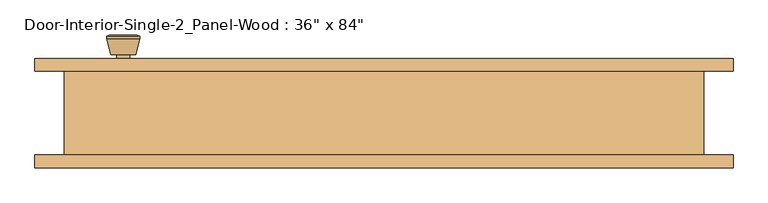
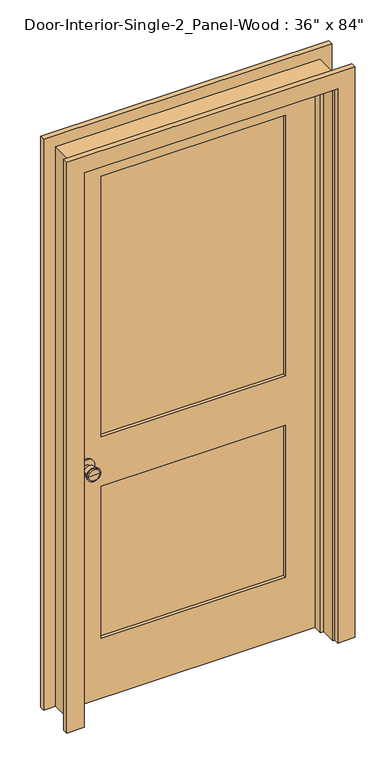
"""IFC4 building model written with IfcOpenShell, lengths in millimetres: door geometry."""

import ifcopenshell
import ifcopenshell.guid

model = None  # the IFC model being written
_history = None  # IfcOwnerHistory: only IFC2X3 demands one
_inside = {}  # id of a spatial element -> (the spatial element, [elements in it])
_under = {}  # id of a project, library or spatial element -> (it, [spatial elements below it])
_declared = {}  # id of a project -> (the project, [libraries it declares])
_typed = {}  # id of a type object -> (the type object, [elements of that type])
_made_of = {}  # id of a material, layer set ... -> (it, [elements and type objects made of it])


def new_model(schema):
    """Start an empty IFC model of exactly this schema.

    Asked for "IFC4X3", IfcOpenShell would pick the latest addendum, in which some entities
    have other attributes; the version numbers below select the first issue.
    IFC2X3 requires an IfcOwnerHistory on every rooted entity: one is made here for all.
    """
    global model, _history
    if schema == "IFC4X3":
        model = ifcopenshell.file(schema_version=(4, 3, 0, 0))
    else:
        model = ifcopenshell.file(schema=schema)
    _inside.clear()
    _under.clear()
    _declared.clear()
    _typed.clear()
    _made_of.clear()
    _history = None
    if model.schema == "IFC2X3":
        org = make("IfcOrganization", Name="unknown")
        user = make(
            "IfcPersonAndOrganization",
            ThePerson=make("IfcPerson", FamilyName="unknown"),
            TheOrganization=org,
        )
        app = make(
            "IfcApplication",
            ApplicationDeveloper=org,
            Version="unknown",
            ApplicationFullName="unknown",
            ApplicationIdentifier="unknown",
        )
        _history = make(
            "IfcOwnerHistory",
            OwningUser=user,
            OwningApplication=app,
            ChangeAction="ADDED",
            CreationDate=0,
        )
    return model


def make(cls, **values):
    """One entity of the class cls with the attributes given. An attribute that is None is left unset."""
    return model.create_entity(
        cls, **{name: value for name, value in values.items() if value is not None}
    )


def rooted(cls, **values):
    """An entity with a GlobalId (a new one), such as an element, a storey or a relation."""
    return make(cls, GlobalId=ifcopenshell.guid.new(), OwnerHistory=_history, **values)


def si_unit(unit_type, name, prefix=None):
    """IfcSIUnit, for example si_unit("LENGTHUNIT", "METRE", prefix="MILLI")."""
    return make("IfcSIUnit", UnitType=unit_type, Prefix=prefix, Name=name)


def assignment(units):
    """IfcUnitAssignment: the units of a project."""
    return None if units is None else make("IfcUnitAssignment", Units=units)


def point(xyz):
    """IfcCartesianPoint."""
    return None if xyz is None else make("IfcCartesianPoint", Coordinates=xyz)


def direction(xyz):
    """IfcDirection."""
    return None if xyz is None else make("IfcDirection", DirectionRatios=xyz)


def frame(location, z_axis=None, x_axis=None):
    """IfcAxis2Placement3D, a coordinate frame: its origin and axes. An axis left out is left unset."""
    return make(
        "IfcAxis2Placement3D",
        Location=point(location),
        Axis=direction(z_axis),
        RefDirection=direction(x_axis),
    )


def frame_2d(location, x_axis=None):
    """IfcAxis2Placement2D, a coordinate frame in the plane: its origin and x axis."""
    return make(
        "IfcAxis2Placement2D", Location=point(location), RefDirection=direction(x_axis)
    )


def origin():
    """The frame at (0, 0, 0) with its axes left unset."""
    return frame((0.0, 0.0, 0.0))


def place(relative_to, where):
    """IfcLocalPlacement: puts the frame where relative to a parent placement (None: the world)."""
    return make(
        "IfcLocalPlacement", PlacementRelTo=relative_to, RelativePlacement=where
    )


def context(
    kind, dimensions, precision=None, world=None, true_north=None, identifier=None
):
    """IfcGeometricRepresentationContext, for example the 3D "Model" context."""
    return make(
        "IfcGeometricRepresentationContext",
        ContextIdentifier=identifier,
        ContextType=kind,
        CoordinateSpaceDimension=dimensions,
        Precision=precision,
        WorldCoordinateSystem=world,
        TrueNorth=true_north,
    )


def project(units=None, contexts=None):
    """IfcProject with its units and contexts."""
    return rooted(
        "IfcProject",
        Name="project",
        RepresentationContexts=contexts,
        UnitsInContext=assignment(units),
    )


def spatial(cls, under=None, at=None, **own):
    """A site, building, storey or space (cls), placed at a placement, below another one or the project."""
    s = rooted(cls, ObjectPlacement=at, **own)
    if under is not None:
        _under.setdefault(under.id(), (under, []))[1].append(s)
    return s


def polyline(points):
    """IfcPolyline through the points."""
    return make("IfcPolyline", Points=[point(p) for p in points])


def circle_curve(where, radius):
    """IfcCircle in the frame where."""
    return make("IfcCircle", Position=where, Radius=radius)


def trimmed(basis, trim1, trim2, sense, master):
    """IfcTrimmedCurve: the piece of a basis curve between two trims."""
    return make(
        "IfcTrimmedCurve",
        BasisCurve=basis,
        Trim1=trim1,
        Trim2=trim2,
        SenseAgreement=sense,
        MasterRepresentation=master,
    )


def segment(curve, same_sense, transition):
    """IfcCompositeCurveSegment."""
    return make(
        "IfcCompositeCurveSegment",
        Transition=transition,
        SameSense=same_sense,
        ParentCurve=curve,
    )


def composite_curve(segments, self_intersect=None):
    """IfcCompositeCurve: segments joined end to end."""
    return make("IfcCompositeCurve", Segments=segments, SelfIntersect=self_intersect)


def outline(outer, holes=None, kind="AREA"):
    """IfcArbitraryClosedProfileDef: a profile drawn as a closed curve; with holes, ...WithVoids."""
    if holes is None:
        return make("IfcArbitraryClosedProfileDef", ProfileType=kind, OuterCurve=outer)
    return make(
        "IfcArbitraryProfileDefWithVoids",
        ProfileType=kind,
        OuterCurve=outer,
        InnerCurves=holes,
    )


def extrude(swept, where, along, depth):
    """IfcExtrudedAreaSolid: the profile swept, set in the frame where, extruded along a direction by depth."""
    return make(
        "IfcExtrudedAreaSolid",
        SweptArea=swept,
        Position=where,
        ExtrudedDirection=direction(along),
        Depth=depth,
    )


def faces_of(points, faces, orient=None, outer=None):
    """IfcFace entities. A face is a list of loops; a loop is a list of indices into points, from 0.

    orient and outer hold one flag for each loop. By default every Orientation is true, the
    first loop of a face is its IfcFaceOuterBound and the others are IfcFaceBound.
    """
    made = []
    for i, loops in enumerate(faces):
        bounds = []
        for j, loop in enumerate(loops):
            is_outer = j == 0 if outer is None else outer[i][j]
            bounds.append(
                make(
                    "IfcFaceOuterBound" if is_outer else "IfcFaceBound",
                    Bound=make("IfcPolyLoop", Polygon=[points[k] for k in loop]),
                    Orientation=True if orient is None else orient[i][j],
                )
            )
        made.append(make("IfcFace", Bounds=bounds))
    return made


def faceted_brep(points, faces, orient=None, outer=None, voids=None):
    """IfcFacetedBrep: a solid bounded by flat faces; with voids (closed shells), ...WithVoids."""
    shared = [point(p) for p in points]
    hull = make("IfcClosedShell", CfsFaces=faces_of(shared, faces, orient, outer))
    if voids is None:
        return make("IfcFacetedBrep", Outer=hull)
    return make(
        "IfcFacetedBrepWithVoids",
        Outer=hull,
        Voids=[
            make(cls, CfsFaces=faces_of(shared, fs, o, b)) for cls, fs, o, b in voids
        ],
    )


def shape(context_of_items, identifier, shape_type, items):
    """IfcShapeRepresentation: the items that make up one representation, for example the "Body"."""
    return make(
        "IfcShapeRepresentation",
        ContextOfItems=context_of_items,
        RepresentationIdentifier=identifier,
        RepresentationType=shape_type,
        Items=items,
    )


def source(mapping_origin, context_of_items, identifier, shape_type, items):
    """IfcRepresentationMap: a shape defined once, which mapped items show again and again."""
    return make(
        "IfcRepresentationMap",
        MappingOrigin=mapping_origin,
        MappedRepresentation=shape(context_of_items, identifier, shape_type, items),
    )


def transform(
    local_origin,
    x_axis=None,
    y_axis=None,
    z_axis=None,
    scale=None,
    scale2=None,
    scale3=None,
    uniform=True,
):
    """IfcCartesianTransformationOperator3D, or its non-uniform kind. x_axis, y_axis, z_axis: its Axis1, 2, 3."""
    if uniform:
        return make(
            "IfcCartesianTransformationOperator3D",
            Axis1=direction(x_axis),
            Axis2=direction(y_axis),
            LocalOrigin=point(local_origin),
            Scale=scale,
            Axis3=direction(z_axis),
        )
    return make(
        "IfcCartesianTransformationOperator3DnonUniform",
        Axis1=direction(x_axis),
        Axis2=direction(y_axis),
        LocalOrigin=point(local_origin),
        Scale=scale,
        Axis3=direction(z_axis),
        Scale2=scale2,
        Scale3=scale3,
    )


def mapped(mapping_source, mapping_target):
    """IfcMappedItem: shows the shape of a source again, moved by a transform."""
    return make(
        "IfcMappedItem", MappingSource=mapping_source, MappingTarget=mapping_target
    )


def made_of(thing, what):
    """Note that an element or type object is made of a material, layer set ...; save() writes the relation."""
    if what is not None:
        _made_of.setdefault(what.id(), (what, []))[1].append(thing)
    return thing


def element(
    cls,
    number,
    at=None,
    inside=None,
    cuts=None,
    type_object=None,
    material=None,
    context=None,
    identifier="Body",
    shape_type=None,
    held_by="IfcProductDefinitionShape",
    body=None,
    shapes=None,
    **own,
):
    """One element of the class cls, such as IfcWall. Its Tag is "e" and its number.

    at: its placement. inside: the storey or other place that contains it. cuts: it is an
    opening in that element (IfcRelVoidsElement). A single representation is given by context,
    identifier, shape_type and body (its items); several are given by shapes. held_by: the class
    of the entity that holds the representations. save() writes the other relations.
    """
    e = rooted(cls, Tag="e%d" % number, ObjectPlacement=at, **own)
    if body is not None:
        shapes = [shape(context, identifier, shape_type, body)]
    if shapes is not None:
        e.Representation = make(held_by, Representations=shapes)
    if inside is not None:
        _inside.setdefault(inside.id(), (inside, []))[1].append(e)
    if cuts is not None:
        rooted(
            "IfcRelVoidsElement", RelatingBuildingElement=cuts, RelatedOpeningElement=e
        )
    if type_object is not None:
        _typed.setdefault(type_object.id(), (type_object, []))[1].append(e)
    return made_of(e, material)


def aggregate(whole, parts):
    """IfcRelAggregates: a whole, such as a stair, and the parts it consists of."""
    return rooted("IfcRelAggregates", RelatingObject=whole, RelatedObjects=parts)


def save(model, path):
    """Write the relations noted so far, then the file.

    IfcRelAggregates (storeys below a building ...), IfcRelContainedInSpatialStructure (elements
    in a storey), IfcRelDefinesByType, IfcRelAssociatesMaterial and IfcRelDeclares: one each for
    every whole, place, type object, material and project.
    """
    for whole, parts in _under.values():
        aggregate(whole, parts)
    for where, things in _inside.values():
        rooted(
            "IfcRelContainedInSpatialStructure",
            RelatedElements=things,
            RelatingStructure=where,
        )
    for kind, things in _typed.values():
        rooted("IfcRelDefinesByType", RelatedObjects=things, RelatingType=kind)
    for what, things in _made_of.values():
        rooted("IfcRelAssociatesMaterial", RelatedObjects=things, RelatingMaterial=what)
    for by, libraries in _declared.values():
        rooted("IfcRelDeclares", RelatingContext=by, RelatedDefinitions=libraries)
    model.write(path)


def plane_surface(at):
    """IfcPlane: the flat surface through the origin of the frame at, square to its z axis."""
    return make("IfcPlane", Position=at)


def cylinder_surface(at, radius):
    """IfcCylindricalSurface: all points at the distance radius from the z axis of the frame at."""
    return make("IfcCylindricalSurface", Position=at, Radius=radius)


def revolved_surface(curve, axis_point, axis_direction):
    """IfcSurfaceOfRevolution: the curve turned about the line through axis_point along axis_direction."""
    return make(
        "IfcSurfaceOfRevolution",
        SweptCurve=make("IfcArbitraryOpenProfileDef", ProfileType="CURVE", Curve=curve),
        AxisPosition=make("IfcAxis1Placement", Location=point(axis_point), Axis=direction(axis_direction)),
    )


def advanced_brep(points, edges, surfaces, faces):
    """IfcAdvancedBrep: a solid bounded by faces that lie on surfaces and meet in shared edges.

    An edge is (start, end): straight between two places in points (the first is 0);
    or (start, end, curve); or (start, end, curve, False) where it runs against its curve.
    A face is (place in surfaces, loops), or (place, loops, False) where it looks against
    its surface's normal. A loop lists edges by number (the first is 1), with a minus sign
    where the edge is run from its end to its start. The first loop is the outer one.
    """
    corners = [point(p) for p in points]
    vertices = [make("IfcVertexPoint", VertexGeometry=c) for c in corners]
    made = []
    for start, end, *more in edges:
        made.append(
            make(
                "IfcEdgeCurve",
                EdgeStart=vertices[start],
                EdgeEnd=vertices[end],
                EdgeGeometry=more[0] if more else make("IfcPolyline", Points=[corners[start], corners[end]]),
                SameSense=more[1] if len(more) > 1 else True,
            )
        )
    hull = []
    for where, loops, *sense in faces:
        bounds = []
        for j, loop in enumerate(loops):
            ring = [make("IfcOrientedEdge", EdgeElement=made[abs(k) - 1], Orientation=k > 0) for k in loop]
            bounds.append(
                make(
                    "IfcFaceOuterBound" if j == 0 else "IfcFaceBound",
                    Bound=make("IfcEdgeLoop", EdgeList=ring),
                    Orientation=True,
                )
            )
        hull.append(make("IfcAdvancedFace", Bounds=bounds, FaceSurface=surfaces[where], SameSense=sense[0] if sense else True))
    return make("IfcAdvancedBrep", Outer=make("IfcClosedShell", CfsFaces=hull))


def door_9f0e9c7d(model_context):
    return source(origin(), model_context, "Body", "SolidModel", [
        advanced_brep(
        [(-393.7, 19.4, 914.4), (-383.7, 19.4, 914.4), (-403.7, 19.4, 914.4), (-373.2241324, -29.6, 914.4), (-393.7, -29.6, 914.4), (-414.1758676, -29.6, 914.4), (-368.7, -27.7721319, 914.4), (-418.7, -27.7721319, 914.4), (-368.7, -24.3084537, 914.4), (-418.7, -24.3084537, 914.4), (-375.063764, 0.4, 914.4), (-412.336236, 0.4, 914.4), (-383.7, 0.4, 914.4), (-403.7, 0.4, 914.4)],
        [
            (0, 1),
            (1, 2, circle_curve(frame((-393.7, 19.4, 914.4), z_axis=(0.0, 1.0, 0.0), x_axis=(-1.0, 0.0, 0.0)), 10.0)),
            (2, 0),
            (2, 1, circle_curve(frame((-393.7, 19.4, 914.4), z_axis=(0.0, 1.0, 0.0), x_axis=(-1.0, 0.0, 0.0)), 10.0)),
            (3, 4),
            (4, 5),
            (5, 3, circle_curve(frame((-393.7, -29.6, 914.4), z_axis=(0.0, -1.0, 0.0), x_axis=(-1.0, 0.0, 0.0)), 20.4758676)),
            (3, 5, circle_curve(frame((-393.7, -29.6, 914.4), z_axis=(0.0, -1.0, 0.0), x_axis=(-1.0, 0.0, 0.0)), 20.4758676)),
            (6, 3),
            (5, 7),
            (7, 6, circle_curve(frame((-393.7, -27.7721319, 914.4), z_axis=(0.0, -1.0, 0.0), x_axis=(-1.0, 0.0, 0.0)), 25.0)),
            (6, 7, circle_curve(frame((-393.7, -27.7721319, 914.4), z_axis=(0.0, -1.0, 0.0), x_axis=(-1.0, 0.0, 0.0)), 25.0)),
            (8, 6),
            (7, 9),
            (9, 8, circle_curve(frame((-393.7, -24.3084537, 914.4), z_axis=(0.0, -1.0, 0.0), x_axis=(-1.0, 0.0, 0.0)), 25.0)),
            (8, 9, circle_curve(frame((-393.7, -24.3084537, 914.4), z_axis=(0.0, -1.0, 0.0), x_axis=(-1.0, 0.0, 0.0)), 25.0)),
            (10, 8),
            (9, 11),
            (11, 10, circle_curve(frame((-393.7, 0.4, 914.4), z_axis=(0.0, -1.0, 0.0), x_axis=(-1.0, 0.0, 0.0)), 18.636236)),
            (10, 11, circle_curve(frame((-393.7, 0.4, 914.4), z_axis=(0.0, -1.0, 0.0), x_axis=(-1.0, 0.0, 0.0)), 18.636236)),
            (12, 10),
            (11, 13),
            (13, 12, circle_curve(frame((-393.7, 0.4, 914.4), z_axis=(0.0, -1.0, 0.0), x_axis=(-1.0, 0.0, 0.0)), 10.0)),
            (12, 13, circle_curve(frame((-393.7, 0.4, 914.4), z_axis=(0.0, -1.0, 0.0), x_axis=(-1.0, 0.0, 0.0)), 10.0)),
            (1, 12),
            (13, 2),
        ],
        [
            plane_surface(frame((-393.7, 19.4, 914.4), z_axis=(0.0, 1.0, 0.0), x_axis=(-1.0, 0.0, 0.0))),
            plane_surface(frame((-393.7, -29.6, 914.4), z_axis=(0.0, -1.0, 0.0), x_axis=(-1.0, 0.0, 0.0))),
            revolved_surface(polyline([(-414.1758676, -29.6, 914.4), (-418.7, -27.7721319, 914.4)]), (-393.7, 19.4, 914.4), (0.0, 1.0, 0.0)),
            cylinder_surface(frame((-393.7, 19.4, 914.4), z_axis=(0.0, 1.0, 0.0), x_axis=(-1.0, 0.0, 0.0)), 25.0),
            revolved_surface(polyline([(-418.7, -24.3084537, 914.4), (-412.336236, 0.4, 914.4)]), (-393.7, 19.4, 914.4), (0.0, 1.0, 0.0)),
            plane_surface(frame((-393.7, 0.4, 914.4), z_axis=(0.0, 1.0, 0.0), x_axis=(-1.0, 0.0, 0.0))),
            cylinder_surface(frame((-393.7, 19.4, 914.4), z_axis=(0.0, 1.0, 0.0), x_axis=(-1.0, 0.0, 0.0)), 10.0),
        ],
        [
            (0, [[1, 2, 3]]),
            (0, [[-3, 4, -1]]),
            (1, [[5, 6, 7]]),
            (1, [[-6, -5, 8]]),
            (2, [[9, -7, 10, 11]]),
            (2, [[-10, -8, -9, 12]]),
            (3, [[13, -11, 14, 15]]),
            (3, [[-14, -12, -13, 16]]),
            (4, [[17, -15, 18, 19]]),
            (4, [[-18, -16, -17, 20]]),
            (5, [[21, -19, 22, 23]]),
            (5, [[-22, -20, -21, 24]]),
            (6, [[25, -23, 26, -2]]),
            (6, [[-26, -24, -25, -4]]),
        ],
    ),
        extrude(outline(composite_curve([segment(trimmed(circle_curve(frame_2d((914.4, -393.7)), 30.0), [point((914.4, -423.7))], [point((914.4, -363.7))], False, "CARTESIAN"), True, "CONTINUOUS"), segment(trimmed(circle_curve(frame_2d((914.4, -393.7)), 30.0), [point((914.4, -363.7))], [point((914.4, -423.7))], False, "CARTESIAN"), True, "CONTINUOUS")], self_intersect=False)), frame((0.0, 19.4, 0.0), z_axis=(0.0, 1.0, 0.0), x_axis=(0.0, 0.0, 1.0)), (0.0, 0.0, 1.0), 6.0),
        advanced_brep(
        [(-393.7, 66.325, 914.4), (-403.7, 66.325, 914.4), (-383.7, 66.325, 914.4), (-373.2241324, 115.325, 914.4), (-414.1758676, 115.325, 914.4), (-393.7, 115.325, 914.4), (-368.7, 113.4971319, 914.4), (-418.7, 113.4971319, 914.4), (-368.7, 110.0334537, 914.4), (-418.7, 110.0334537, 914.4), (-375.063764, 85.325, 914.4), (-412.336236, 85.325, 914.4), (-383.7, 85.325, 914.4), (-403.7, 85.325, 914.4)],
        [
            (0, 1),
            (1, 2, circle_curve(frame((-393.7, 66.325, 914.4), z_axis=(0.0, -1.0, 0.0), x_axis=(-1.0, 0.0, 0.0)), 10.0)),
            (2, 0),
            (2, 1, circle_curve(frame((-393.7, 66.325, 914.4), z_axis=(0.0, -1.0, 0.0), x_axis=(-1.0, 0.0, 0.0)), 10.0)),
            (3, 4, circle_curve(frame((-393.7, 115.325, 914.4), z_axis=(0.0, 1.0, 0.0), x_axis=(-1.0, 0.0, 0.0)), 20.4758676)),
            (4, 5),
            (5, 3),
            (4, 3, circle_curve(frame((-393.7, 115.325, 914.4), z_axis=(0.0, 1.0, 0.0), x_axis=(-1.0, 0.0, 0.0)), 20.4758676)),
            (6, 7, circle_curve(frame((-393.7, 113.4971319, 914.4), z_axis=(0.0, 1.0, 0.0), x_axis=(-1.0, 0.0, 0.0)), 25.0)),
            (7, 4),
            (3, 6),
            (7, 6, circle_curve(frame((-393.7, 113.4971319, 914.4), z_axis=(0.0, 1.0, 0.0), x_axis=(-1.0, 0.0, 0.0)), 25.0)),
            (8, 9, circle_curve(frame((-393.7, 110.0334537, 914.4), z_axis=(0.0, 1.0, 0.0), x_axis=(-1.0, 0.0, 0.0)), 25.0)),
            (9, 7),
            (6, 8),
            (9, 8, circle_curve(frame((-393.7, 110.0334537, 914.4), z_axis=(0.0, 1.0, 0.0), x_axis=(-1.0, 0.0, 0.0)), 25.0)),
            (10, 11, circle_curve(frame((-393.7, 85.325, 914.4), z_axis=(0.0, 1.0, 0.0), x_axis=(-1.0, 0.0, 0.0)), 18.636236)),
            (11, 9),
            (8, 10),
            (11, 10, circle_curve(frame((-393.7, 85.325, 914.4), z_axis=(0.0, 1.0, 0.0), x_axis=(-1.0, 0.0, 0.0)), 18.636236)),
            (12, 13, circle_curve(frame((-393.7, 85.325, 914.4), z_axis=(0.0, 1.0, 0.0), x_axis=(-1.0, 0.0, 0.0)), 10.0)),
            (13, 11),
            (10, 12),
            (13, 12, circle_curve(frame((-393.7, 85.325, 914.4), z_axis=(0.0, 1.0, 0.0), x_axis=(-1.0, 0.0, 0.0)), 10.0)),
            (1, 13),
            (12, 2),
        ],
        [
            plane_surface(frame((-393.7, 66.325, 914.4), z_axis=(0.0, -1.0, 0.0), x_axis=(-1.0, 0.0, 0.0))),
            plane_surface(frame((-393.7, 115.325, 914.4), z_axis=(0.0, 1.0, 0.0), x_axis=(-1.0, 0.0, 0.0))),
            revolved_surface(polyline([(-414.1758676, 115.325, 914.4), (-418.7, 113.4971319, 914.4)]), (-393.7, 66.325, 914.4), (0.0, -1.0, 0.0)),
            cylinder_surface(frame((-393.7, 66.325, 914.4), z_axis=(0.0, -1.0, 0.0), x_axis=(-1.0, 0.0, 0.0)), 25.0),
            revolved_surface(polyline([(-418.7, 110.0334537, 914.4), (-412.336236, 85.325, 914.4)]), (-393.7, 66.325, 914.4), (0.0, -1.0, 0.0)),
            plane_surface(frame((-393.7, 85.325, 914.4), z_axis=(0.0, -1.0, 0.0), x_axis=(-1.0, 0.0, 0.0))),
            cylinder_surface(frame((-393.7, 66.325, 914.4), z_axis=(0.0, -1.0, 0.0), x_axis=(-1.0, 0.0, 0.0)), 10.0),
        ],
        [
            (0, [[1, 2, 3]]),
            (0, [[-3, 4, -1]]),
            (1, [[5, 6, 7]]),
            (1, [[8, -7, -6]]),
            (2, [[9, 10, -5, 11]]),
            (2, [[12, -11, -8, -10]]),
            (3, [[13, 14, -9, 15]]),
            (3, [[16, -15, -12, -14]]),
            (4, [[17, 18, -13, 19]]),
            (4, [[20, -19, -16, -18]]),
            (5, [[21, 22, -17, 23]]),
            (5, [[24, -23, -20, -22]]),
            (6, [[-2, 25, -21, 26]]),
            (6, [[-4, -26, -24, -25]]),
        ],
    ),
        extrude(outline(composite_curve([segment(trimmed(circle_curve(frame_2d((914.4, -393.7)), 30.0), [point((914.4, -423.7))], [point((914.4, -363.7))], False, "CARTESIAN"), True, "CONTINUOUS"), segment(trimmed(circle_curve(frame_2d((914.4, -393.7)), 30.0), [point((914.4, -363.7))], [point((914.4, -423.7))], False, "CARTESIAN"), True, "CONTINUOUS")], self_intersect=False)), frame((0.0, 60.325, 0.0), z_axis=(0.0, 1.0, 0.0), x_axis=(0.0, 0.0, 1.0)), (0.0, 0.0, 1.0), 6.0),
        extrude(outline(polyline([(336.55, 37.0416667), (-336.55, 37.0416667), (-336.55, 48.6833333), (336.55, 48.6833333), (336.55, 37.0416667)])), frame((0.0, 0.0, 1009.65), z_axis=(0.0, 0.0, 1.0), x_axis=(1.0, 0.0, 0.0)), (0.0, 0.0, 1.0), 1004.8875),
        extrude(outline(polyline([(336.55, 37.0416667), (-336.55, 37.0416667), (-336.55, 48.6833333), (336.55, 48.6833333), (336.55, 37.0416667)])), frame((0.0, 0.0, 231.775), z_axis=(0.0, 0.0, 1.0), x_axis=(1.0, 0.0, 0.0)), (0.0, 0.0, 1.0), 587.375),
        extrude(outline(polyline([(2133.6, -457.2), (0.0, -457.2), (0.0, 457.2), (2133.6, 457.2), (2133.6, -457.2)]), holes=[polyline([(2014.5375, -336.55), (2014.5375, 336.55), (1009.65, 336.55), (1009.65, -336.55), (2014.5375, -336.55)]), polyline([(819.15, -336.55), (819.15, 336.55), (231.775, 336.55), (231.775, -336.55), (819.15, -336.55)])]), frame((0.0, 25.4, 0.0), z_axis=(0.0, 1.0, 0.0), x_axis=(0.0, 0.0, 1.0)), (0.0, 0.0, 1.0), 34.925),
        faceted_brep([(482.6, 60.325, 0.0), (482.6, -66.675, 0.0), (457.2, -66.675, 0.0), (457.2, -9.525, 0.0), (444.5, -9.525, 0.0), (444.5, 25.4, 0.0), (457.2, 25.4, 0.0), (457.2, 60.325, 0.0), (482.6, 60.325, 2159.0), (482.6, -66.675, 2159.0), (-482.6, -66.675, 2159.0), (-482.6, -66.675, 0.0), (-457.2, -66.675, 0.0), (-457.2, -66.675, 2133.6), (457.2, -66.675, 2133.6), (457.2, -9.525, 2133.6), (-457.2, -9.525, 2133.6), (-457.2, -9.525, 0.0), (-444.5, -9.525, 0.0), (-444.5, -9.525, 2120.9), (444.5, -9.525, 2120.9), (444.5, 25.4, 2120.9), (-444.5, 25.4, 2120.9), (-444.5, 25.4, 0.0), (-457.2, 25.4, 0.0), (-457.2, 25.4, 2133.6), (457.2, 25.4, 2133.6), (457.2, 60.325, 2133.6), (-457.2, 60.325, 2133.6), (-457.2, 60.325, 0.0), (-482.6, 60.325, 0.0), (-482.6, 60.325, 2159.0)], [[[0, 1, 2, 3, 4, 5, 6, 7]], [[1, 0, 8, 9]], [[2, 1, 9, 10, 11, 12, 13, 14]], [[3, 2, 14, 15]], [[4, 3, 15, 16, 17, 18, 19, 20]], [[5, 4, 20, 21]], [[6, 5, 21, 22, 23, 24, 25, 26]], [[7, 6, 26, 27]], [[0, 7, 27, 28, 29, 30, 31, 8]], [[9, 8, 31, 10]], [[15, 14, 13, 16]], [[21, 20, 19, 22]], [[27, 26, 25, 28]], [[30, 29, 24, 23, 18, 17, 12, 11]], [[10, 31, 30, 11]], [[16, 13, 12, 17]], [[22, 19, 18, 23]], [[28, 25, 24, 29]]]),
        extrude(outline(polyline([(0.0, 463.55), (0.0, 527.05), (2203.45, 527.05), (2203.45, -527.05), (0.0, -527.05), (0.0, -463.55), (2139.95, -463.55), (2139.95, 463.55), (0.0, 463.55)])), frame((0.0, -85.725, 0.0), z_axis=(0.0, 1.0, 0.0), x_axis=(0.0, 0.0, 1.0)), (0.0, 0.0, 1.0), 19.05),
        extrude(outline(polyline([(0.0, 463.55), (0.0, 527.05), (2203.45, 527.05), (2203.45, -527.05), (0.0, -527.05), (0.0, -463.55), (2139.95, -463.55), (2139.95, 463.55), (0.0, 463.55)])), frame((0.0, 60.325, 0.0), z_axis=(0.0, 1.0, 0.0), x_axis=(0.0, 0.0, 1.0)), (0.0, 0.0, 1.0), 19.05),
    ])


if __name__ == "__main__":
    model = new_model("IFC4")
    model_context = context("Model", 3, world=origin())
    ifc_project = project(units=[si_unit("LENGTHUNIT", "METRE", prefix="MILLI")], contexts=[model_context])
    site = spatial("IfcSite", under=ifc_project)
    building = spatial("IfcBuilding", under=site)
    placement = place(None, origin())
    door_shape = door_9f0e9c7d(model_context)
    element("IfcDoor", 1, ObjectType="Door-Interior-Single-2_Panel-Wood : 36\" x 84\"", at=placement, inside=building, context=model_context, shape_type="MappedRepresentation", body=[
        mapped(door_shape, transform((0.0, 0.0, 0.0), x_axis=(1.0, 0.0, 0.0), y_axis=(0.0, 1.0, 0.0), z_axis=(0.0, 0.0, 1.0))),
    ])
    save(model, "model.ifc")

# Revit data of these elements
# Type "Door-Interior-Single-2_Panel-Wood : 36\" x 84\""
#   Type Mark = "17"
#   Assembly Code = "C1020300"
#   Analytic Construction = "Wooden"
#   Top Rail = 0' - 4 11/16"
#   Thickness = 0' - 1 3/8"
#   Thermal Resistance (R) = 2.5876 (h·ft²·°F)/BTU
#   Swing Angle [instance default] = 90.00°
#   Stiles = 0' - 4 3/4"
#   Rough Width = 3' - 2"
#   Rough Height = 7' - 1"
#   Lock Rail = 0' - 7 1/2"
#   Height = 7' - 0"
#   Width = 3' - 0"
#   Heat Transfer Coefficient (U) = 0.3865 BTU/(h·ft²·°F)
#   Bottom Rail = 0' - 9 1/8"
#   Function = 0
#   Define Thermal Properties by = 1
#   Trim Material = Cherry
#   Panel Material = Cherry
#   Frame Material = Cherry
#   Door Handle Material = Aluminum
#   Visual Light Transmittance = 0
#   Solar Heat Gain Coefficient = 0
#   Wall Closure = (empty or 0)
#   Function = (empty or 0)
# Element 1 (IfcDoor, "Door-Interior-Single-2_Panel-Wood : 36\" x 84\"")
#   Materials on its faces: "Cherry", "Aluminum"
# Materials
#   "Cherry": class "Wood", colour RGB 157 77 38, transparency 0, Description = "Prunus Serotina", Cost = 0
#   "Aluminum": class "Metal", colour RGB 120 120 120, transparency 0, Description = "Aluminum 6061", Cost = 0
